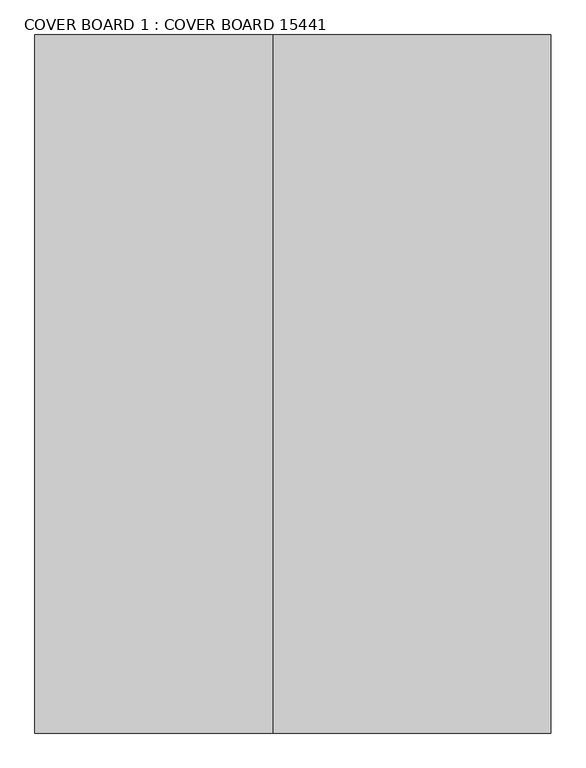
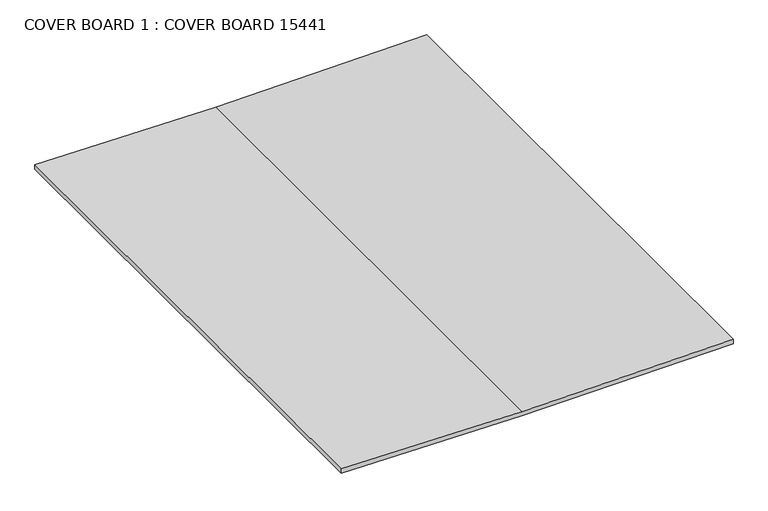
"""IFC4 building model written with IfcOpenShell, lengths in millimetres: proxy geometry, COVER BOARD 1 : COVER BOARD 15441."""

from ifc_helpers import new_model, si_unit, frame, origin, place, context, project, spatial, polyline, outline, extrude, source, transform, mapped, element, save


def cover_board_1_cover_board_15441_a2131a35(model_context):
    return source(origin(), model_context, "Body", "SweptSolid", [
        extrude(outline(polyline([(40228.1021556, -1886.5629484), (40237.9000089, -2567.3737014), (40220.5682898, -2567.3737014), (40210.7704365, -1886.5629484), (40220.5682898, -1090.0815411), (40237.9000089, -1090.0815411), (40228.1021556, -1886.5629484)])), frame((0.0, -1052.6406573, 0.0), z_axis=(0.0, 1.0, 0.0), x_axis=(0.0, 0.0, 1.0)), (0.0, 0.0, 1.0), 2000.0),
    ])


if __name__ == "__main__":
    model = new_model("IFC4")
    model_context = context("Model", 3, world=origin())
    ifc_project = project(units=[si_unit("LENGTHUNIT", "METRE", prefix="MILLI")], contexts=[model_context])
    site = spatial("IfcSite", under=ifc_project)
    building = spatial("IfcBuilding", under=site)
    placement = place(None, origin())
    cover_board_1_cover_board_15441_shape = cover_board_1_cover_board_15441_a2131a35(model_context)
    element("IfcBuildingElementProxy", 1, Name="COVER BOARD 1 : COVER BOARD 15441", ObjectType="COVER BOARD 1 : COVER BOARD 15441", at=placement, inside=building, context=model_context, shape_type="MappedRepresentation", body=[
        mapped(cover_board_1_cover_board_15441_shape, transform((0.0, 0.0, 0.0), x_axis=(1.0, 0.0, 0.0), y_axis=(0.0, 1.0, 0.0), z_axis=(0.0, 0.0, 1.0))),
    ])
    save(model, "model.ifc")

# Revit data of these elements
# Type "COVER BOARD 1 : COVER BOARD 15441"
#   NameOverride = "COVER BOARD"
# Element 1 (IfcBuildingElementProxy, "COVER BOARD 1 : COVER BOARD 15441")
#   Materials on its faces: "CDX PLYWOOD - SEE STRUCTURAL DWGS"
# Materials
#   "CDX PLYWOOD - SEE STRUCTURAL DWGS": class "Unassigned", colour RGB 202 163 108, transparency 0, Cost = 0
